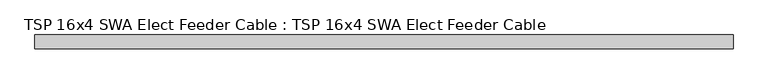
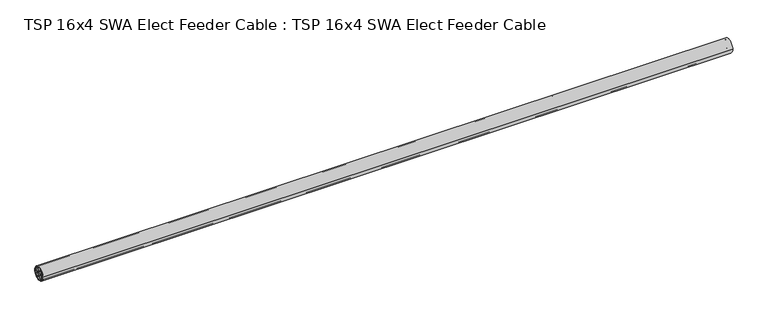
"""IFC4 building model written with IfcOpenShell, lengths in millimetres: proxy geometry, TSP 16x4 SWA Elect Feeder Cable : TSP 16x4 SWA Elect Feeder Cable."""

from ifc_helpers import new_model, si_unit, point, frame, frame_2d, origin, origin_2d, place, context, project, spatial, circle_curve, trimmed, segment, composite_curve, outline, extrude, source, transform, mapped, element, save


def tsp_16x4_swa_elect_feeder_cable_tsp_16x4_swa_elect_feeder_19b787d1(model_context):
    return source(origin(), model_context, "Body", "SweptSolid", [
        extrude(outline(composite_curve([segment(trimmed(circle_curve(origin_2d(), 30.0), [point((-30.0, 0.0))], [point((30.0, 0.0))], False, "CARTESIAN"), True, "CONTINUOUS"), segment(trimmed(circle_curve(origin_2d(), 30.0), [point((30.0, 0.0))], [point((-30.0, 0.0))], False, "CARTESIAN"), True, "CONTINUOUS")], self_intersect=False), holes=[composite_curve([segment(trimmed(circle_curve(origin_2d(), 27.0), [point((-27.0, 0.0))], [point((27.0, 0.0))], True, "CARTESIAN"), True, "CONTINUOUS"), segment(trimmed(circle_curve(origin_2d(), 27.0), [point((27.0, 0.0))], [point((-27.0, 0.0))], True, "CARTESIAN"), True, "CONTINUOUS")], self_intersect=False)]), frame((0.0, 0.0, 0.0), z_axis=(1.0, 0.0, 0.0), x_axis=(0.0, 1.0, 0.0)), (0.0, 0.0, 1.0), 3000.0),
        extrude(outline(composite_curve([segment(trimmed(circle_curve(frame_2d((11.691343, 10.1)), 8.0), [point((3.691343, 10.1))], [point((19.691343, 10.1))], False, "CARTESIAN"), True, "CONTINUOUS"), segment(trimmed(circle_curve(frame_2d((11.691343, 10.1)), 8.0), [point((19.691343, 10.1))], [point((3.691343, 10.1))], False, "CARTESIAN"), True, "CONTINUOUS")], self_intersect=False)), frame((0.0, 0.0, 0.0), z_axis=(1.0, 0.0, 0.0), x_axis=(0.0, 1.0, 0.0)), (0.0, 0.0, 1.0), 3000.0),
        extrude(outline(composite_curve([segment(trimmed(circle_curve(frame_2d((-11.691343, 10.1)), 8.0), [point((-19.691343, 10.1))], [point((-3.691343, 10.1))], False, "CARTESIAN"), True, "CONTINUOUS"), segment(trimmed(circle_curve(frame_2d((-11.691343, 10.1)), 8.0), [point((-3.691343, 10.1))], [point((-19.691343, 10.1))], False, "CARTESIAN"), True, "CONTINUOUS")], self_intersect=False)), frame((0.0, 0.0, 0.0), z_axis=(1.0, 0.0, 0.0), x_axis=(0.0, 1.0, 0.0)), (0.0, 0.0, 1.0), 3000.0),
        extrude(outline(composite_curve([segment(trimmed(circle_curve(frame_2d((-11.691343, -10.1)), 8.0), [point((-19.691343, -10.1))], [point((-3.691343, -10.1))], False, "CARTESIAN"), True, "CONTINUOUS"), segment(trimmed(circle_curve(frame_2d((-11.691343, -10.1)), 8.0), [point((-3.691343, -10.1))], [point((-19.691343, -10.1))], False, "CARTESIAN"), True, "CONTINUOUS")], self_intersect=False)), frame((0.0, 0.0, 0.0), z_axis=(1.0, 0.0, 0.0), x_axis=(0.0, 1.0, 0.0)), (0.0, 0.0, 1.0), 3000.0),
        extrude(outline(composite_curve([segment(trimmed(circle_curve(frame_2d((11.691343, -10.1)), 8.0), [point((3.691343, -10.1))], [point((19.691343, -10.1))], False, "CARTESIAN"), True, "CONTINUOUS"), segment(trimmed(circle_curve(frame_2d((11.691343, -10.1)), 8.0), [point((19.691343, -10.1))], [point((3.691343, -10.1))], False, "CARTESIAN"), True, "CONTINUOUS")], self_intersect=False)), frame((0.0, 0.0, 0.0), z_axis=(1.0, 0.0, 0.0), x_axis=(0.0, 1.0, 0.0)), (0.0, 0.0, 1.0), 3000.0),
        extrude(outline(composite_curve([segment(trimmed(circle_curve(origin_2d(), 27.0), [point((27.0, 0.0))], [point((-27.0, 0.0))], False, "CARTESIAN"), True, "CONTINUOUS"), segment(trimmed(circle_curve(origin_2d(), 27.0), [point((-27.0, 0.0))], [point((27.0, 0.0))], False, "CARTESIAN"), True, "CONTINUOUS")], self_intersect=False), holes=[composite_curve([segment(trimmed(circle_curve(frame_2d((-11.691343, 10.1)), 8.0), [point((-3.691343, 10.1))], [point((-19.691343, 10.1))], True, "CARTESIAN"), True, "CONTINUOUS"), segment(trimmed(circle_curve(frame_2d((-11.691343, 10.1)), 8.0), [point((-19.691343, 10.1))], [point((-3.691343, 10.1))], True, "CARTESIAN"), True, "CONTINUOUS")], self_intersect=False), composite_curve([segment(trimmed(circle_curve(frame_2d((11.691343, 10.1)), 8.0), [point((3.691343, 10.1))], [point((19.691343, 10.1))], True, "CARTESIAN"), True, "CONTINUOUS"), segment(trimmed(circle_curve(frame_2d((11.691343, 10.1)), 8.0), [point((19.691343, 10.1))], [point((3.691343, 10.1))], True, "CARTESIAN"), True, "CONTINUOUS")], self_intersect=False), composite_curve([segment(trimmed(circle_curve(frame_2d((-11.691343, -10.15)), 8.0), [point((-19.691343, -10.15))], [point((-3.691343, -10.15))], True, "CARTESIAN"), True, "CONTINUOUS"), segment(trimmed(circle_curve(frame_2d((-11.691343, -10.15)), 8.0), [point((-3.691343, -10.15))], [point((-19.691343, -10.15))], True, "CARTESIAN"), True, "CONTINUOUS")], self_intersect=False), composite_curve([segment(trimmed(circle_curve(frame_2d((11.691343, -10.15)), 8.0), [point((3.691343, -10.15))], [point((19.691343, -10.15))], True, "CARTESIAN"), True, "CONTINUOUS"), segment(trimmed(circle_curve(frame_2d((11.691343, -10.15)), 8.0), [point((19.691343, -10.15))], [point((3.691343, -10.15))], True, "CARTESIAN"), True, "CONTINUOUS")], self_intersect=False)]), frame((0.0, 0.0, 0.0), z_axis=(1.0, 0.0, 0.0), x_axis=(0.0, 1.0, 0.0)), (0.0, 0.0, 1.0), 3000.0),
    ])


if __name__ == "__main__":
    model = new_model("IFC4")
    model_context = context("Model", 3, world=origin())
    ifc_project = project(units=[si_unit("LENGTHUNIT", "METRE", prefix="MILLI")], contexts=[model_context])
    site = spatial("IfcSite", under=ifc_project)
    building = spatial("IfcBuilding", under=site)
    placement = place(None, origin())
    tsp_16x4_swa_elect_feeder_cable_tsp_16x4_swa_elect_feeder_shape = tsp_16x4_swa_elect_feeder_cable_tsp_16x4_swa_elect_feeder_19b787d1(model_context)
    element("IfcBuildingElementProxy", 1, Name="TSP 16x4 SWA Elect Feeder Cable : TSP 16x4 SWA Elect Feeder Cable", ObjectType="TSP 16x4 SWA Elect Feeder Cable : TSP 16x4 SWA Elect Feeder Cable", at=placement, inside=building, context=model_context, shape_type="MappedRepresentation", body=[
        mapped(tsp_16x4_swa_elect_feeder_cable_tsp_16x4_swa_elect_feeder_shape, transform((0.0, 0.0, 0.0), x_axis=(1.0, 0.0, 0.0), y_axis=(0.0, 1.0, 0.0), z_axis=(0.0, 0.0, 1.0))),
    ])
    save(model, "model.ifc")

# Revit data of these elements
# Type "TSP 16x4 SWA Elect Feeder Cable : TSP 16x4 SWA Elect Feeder Cable"
#   Model = "TSP_ELECSC164"
#   built-in parameter 1001306 [instance default] = 5.24934 (stored number, unit not read)
#   Cable Length [instance default] = 1600 mm
#   Default Elevation = 0
# Element 1 (IfcBuildingElementProxy, "TSP 16x4 SWA Elect Feeder Cable : TSP 16x4 SWA Elect Feeder Cable")
#   built-in parameter 1001306 = 9.84252 (stored number, unit not read)
#   Cable Length = 3000 mm
#   Materials on its faces: "Cellulose Fill", "Copper", "Laminate, Red, Matte"
# Materials
#   "Cellulose Fill": class "Generic", colour RGB 0 0 0, transparency 0, Description = "Cellulose loose fill", Cost = 0
#   "Copper": class "Metal", colour RGB 0 0 0, transparency 0, Description = "Copper, matte finish", Cost = 0
#   "Laminate, Red, Matte": class "Plastic", colour RGB 255 0 0, transparency 0, Description = "Plastic Laminate - Red, Matte", Cost = 0
